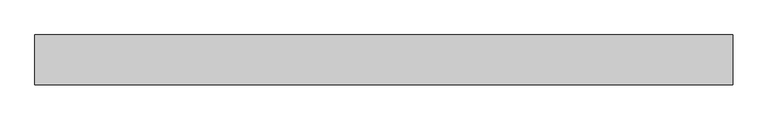
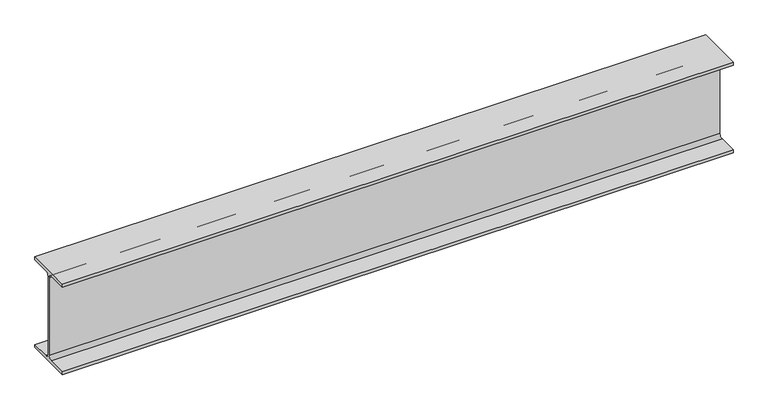
"""IFC4 building model written with IfcOpenShell, lengths in millimetres: beam geometry, 0912_Steel Framing_H-KSD3502 : H_SB_ASB_H-350x175x7x11."""

from ifc_helpers import new_model, si_unit, point, frame, frame_2d, origin, place, context, project, spatial, polyline, circle_curve, trimmed, segment, composite_curve, outline, extrude, source, transform, mapped, element, save


def beam_8a01b06a(model_context):
    return source(origin(), model_context, "Body", "SweptSolid", [
        extrude(outline(composite_curve([segment(polyline([(87.5, -164.0), (87.5, -175.0), (-87.5, -175.0), (-87.5, -164.0), (-17.5, -164.0)]), True, "CONTINUOUS"), segment(trimmed(circle_curve(frame_2d((-17.5, -150.0)), 14.0), [point((-17.5, -164.0))], [point((-3.5, -150.0))], True, "CARTESIAN"), True, "CONTINUOUS"), segment(polyline([(-3.5, -150.0), (-3.5, 150.0)]), True, "CONTINUOUS"), segment(trimmed(circle_curve(frame_2d((-17.5, 150.0)), 14.0), [point((-3.5, 150.0))], [point((-17.5, 164.0))], True, "CARTESIAN"), True, "CONTINUOUS"), segment(polyline([(-17.5, 164.0), (-87.5, 164.0), (-87.5, 175.0), (87.5, 175.0), (87.5, 164.0), (17.5, 164.0)]), True, "CONTINUOUS"), segment(trimmed(circle_curve(frame_2d((17.5, 150.0)), 14.0), [point((17.5, 164.0))], [point((3.5, 150.0))], True, "CARTESIAN"), True, "CONTINUOUS"), segment(polyline([(3.5, 150.0), (3.5, -150.0)]), True, "CONTINUOUS"), segment(trimmed(circle_curve(frame_2d((17.5, -150.0)), 14.0), [point((3.5, -150.0))], [point((17.5, -164.0))], True, "CARTESIAN"), True, "CONTINUOUS"), segment(polyline([(17.5, -164.0), (87.5, -164.0)]), True, "CONTINUOUS")], self_intersect=False)), frame((-1160.5135857, 0.0, 0.0), z_axis=(1.0, 0.0, 0.0), x_axis=(0.0, 1.0, 0.0)), (0.0, 0.0, 1.0), 2456.2874909),
    ])


if __name__ == "__main__":
    model = new_model("IFC4")
    model_context = context("Model", 3, world=origin())
    ifc_project = project(units=[si_unit("LENGTHUNIT", "METRE", prefix="MILLI")], contexts=[model_context])
    site = spatial("IfcSite", under=ifc_project)
    building = spatial("IfcBuilding", under=site)
    placement = place(None, origin())
    beam_shape = beam_8a01b06a(model_context)
    element("IfcBeam", 1, ObjectType="0912_Steel Framing_H-KSD3502 : H_SB_ASB_H-350x175x7x11", at=placement, inside=building, context=model_context, shape_type="MappedRepresentation", body=[
        mapped(beam_shape, transform((0.0, 0.0, 0.0), x_axis=(1.0, 0.0, 0.0), y_axis=(0.0, 1.0, 0.0), z_axis=(0.0, 0.0, 1.0))),
    ])
    save(model, "model.ifc")

# Revit data of these elements
# Type "0912_Steel Framing_H-KSD3502 : H_SB_ASB_H-350x175x7x11"
#   H_WM Code_1 = "S01AA002-00001 | Main Steel Structure Fabrication Work | Shelter/Building | Medium Steel - Standard (90KG/M>Weight≥30KG/M) | Material: (   )"
#   H_WM Code_2 = "S03AA028-00001 | Main Steel Structure Erection Work | Shelter/Building | Medium Steel (90KG/M>Weight≥30KG/M) | Material: (   )"
#   H_WM Code_3 = "S01AA010-00001 | Main Steel Structure Fabrication Work | Shelter/Building | Steel Painting/Coating | for Non-Fireproofed Steel Surface, Surface Preparation, Primer, Second & Final Coat | Material: (   )"
#   H_Q'ty Cal Type Tag = "SB-Q2"
#   Width = 17.5 cm
#   Web Thickness = 0.7 cm
#   Web Fillet = 1.4 cm
#   Warping Constant = 282000.0 cm⁶
#   W = 0
#   Torsional Moment of Inertia = 19.4042 cm⁴
#   Section Area = 63.14 cm²
#   Plastic Modulus weak axis = 174.0 cm³
#   Plastic Modulus strong axis = 868.0 cm³
#   Perimeter = 1.36 m²/m
#   Nominal Weight = 49.60 kgf/m
#   Moment of Inertia weak axis = 984.00 cm⁴
#   Moment of Inertia strong axis = 13600.00 cm⁴
#   Height = 35.0 cm
#   Flange Thickness = 1.1 cm
#   Elastic Modulus weak axis = 112.0 cm³
#   Elastic Modulus strong axis = 775.0 cm³
#   Centroid Vertical = 17.5 cm
#   Centroid Horizontal = 8.75 cm
#   Ix = 136000000
#   Length [instance default] = 1.5240 m
#   Zx = 868000
#   b = 0.1750 m
#   h = 0.3500 m
#   r = 0.0140 m
#   s = 0.0070 m
#   t = 0.0110 m
#   A = 0.006314 m²
#   Structural Material [instance default] = Steel, 45-345
#   Assembly Code = ""
# Element 1 (IfcBeam, "0912_Steel Framing_H-KSD3502 : H_SB_ASB_H-350x175x7x11")
#   Structural Material = none
# Materials
#   "Steel, 45-345": class "Metal", colour RGB 189 187 185, transparency 0, Description = "Steel 345 MPa", Cost = 0
